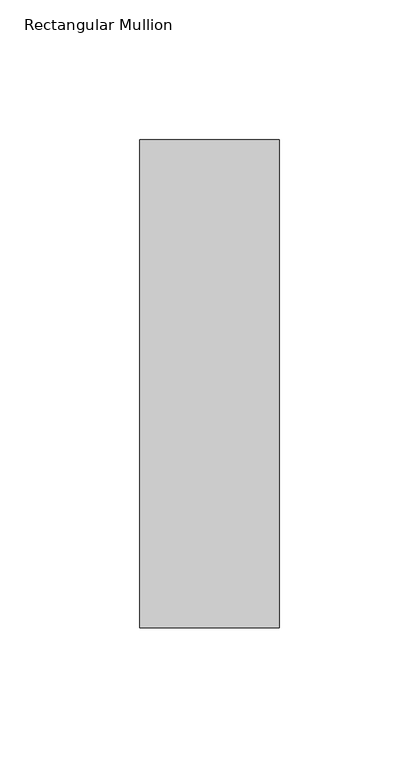
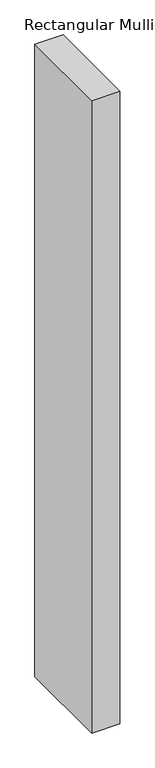
"""IFC4 building model written with IfcOpenShell, lengths in millimetres: member geometry, Rectangular Mullion : WWm-50x175-50mmOffset."""

from ifc_helpers import new_model, si_unit, frame, origin, place, context, project, spatial, polyline, outline, extrude, source, transform, mapped, element, save


def rectangular_mullion_e97ce97f(model_context):
    return source(origin(), model_context, "Body", "SweptSolid", [
        extrude(outline(polyline([(0.0, 87.5), (0.0, -87.5), (-50.0, -87.5), (-50.0, 87.5), (0.0, 87.5)])), frame((0.0, 0.0, -1189.2211826), z_axis=(0.0, 0.0, 1.0), x_axis=(1.0, 0.0, 0.0)), (0.0, 0.0, 1.0), 1189.2211826),
    ])


if __name__ == "__main__":
    model = new_model("IFC4")
    model_context = context("Model", 3, world=origin())
    ifc_project = project(units=[si_unit("LENGTHUNIT", "METRE", prefix="MILLI")], contexts=[model_context])
    site = spatial("IfcSite", under=ifc_project)
    building = spatial("IfcBuilding", under=site)
    placement = place(None, origin())
    rectangular_mullion_shape = rectangular_mullion_e97ce97f(model_context)
    element("IfcMember", 1, ObjectType="Rectangular Mullion : WWm-50x175-50mmOffset", at=placement, inside=building, context=model_context, shape_type="MappedRepresentation", body=[
        mapped(rectangular_mullion_shape, transform((0.0, 0.0, 0.0), x_axis=(1.0, 0.0, 0.0), y_axis=(0.0, 1.0, 0.0), z_axis=(0.0, 0.0, 1.0))),
    ])
    save(model, "model.ifc")

# Revit data of these elements
# Type "Rectangular Mullion : WWm-50x175-50mmOffset"
#   built-in parameter 1007304 = 0.574147 (stored number, unit not read)
#   built-in parameter 1007301 = 0.082021 (stored number, unit not read)
#   built-in parameter 1007300 = 0.082021 (stored number, unit not read)
# Element 1 (IfcMember, "Rectangular Mullion : WWm-50x175-50mmOffset")
#   Materials on its faces: "WW-EC-RGB-Mullion"
# Materials
#   "WW-EC-RGB-Mullion": class "Generic", colour RGB 255 255 255, transparency 0, Comments = "If region requests black mullions, switch asset color to RGB 25-25-25", Description = "Generic Color", Cost = 0
